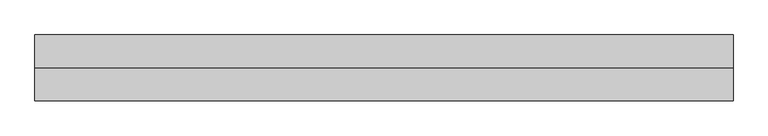
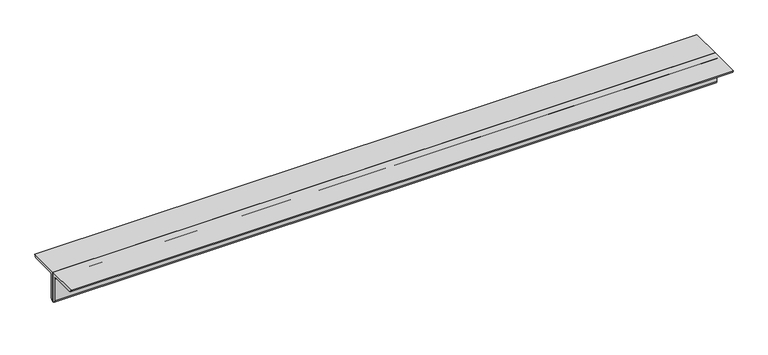
"""IFC4 building model written with IfcOpenShell, lengths in millimetres: beam geometry, 0123_Steel Framing_2Ls-KSD3502 : H_SB_AR_S04_2Ls-130x130x12_VBR1."""

from ifc_helpers import new_model, si_unit, point, frame, frame_2d, origin, place, context, project, spatial, polyline, circle_curve, trimmed, segment, composite_curve, outline, extrude, source, transform, mapped, element, save


def beam_630e65bb(model_context):
    return source(origin(), model_context, "Body", "SweptSolid", [
        extrude(outline(composite_curve([segment(polyline([(0.0, 36.4), (130.0, 36.4)]), True, "CONTINUOUS"), segment(trimmed(circle_curve(frame_2d((118.0, 36.4)), 12.0), [point((130.0, 36.4))], [point((118.0, 24.4))], False, "CARTESIAN"), True, "CONTINUOUS"), segment(polyline([(118.0, 24.4), (24.0, 24.4)]), True, "CONTINUOUS"), segment(trimmed(circle_curve(frame_2d((24.0, 12.4)), 12.0), [point((24.0, 24.4))], [point((12.0, 12.4))], True, "CARTESIAN"), True, "CONTINUOUS"), segment(polyline([(12.0, 12.4), (12.0, -81.6)]), True, "CONTINUOUS"), segment(trimmed(circle_curve(frame_2d((0.0, -81.6)), 12.0), [point((12.0, -81.6))], [point((0.0, -93.6))], False, "CARTESIAN"), True, "CONTINUOUS"), segment(polyline([(0.0, -93.6), (0.0, 36.4)]), True, "CONTINUOUS")], self_intersect=False)), frame((-1375.4177251, 0.0, 0.0), z_axis=(1.0, 0.0, 0.0), x_axis=(0.0, 1.0, 0.0)), (0.0, 0.0, 1.0), 2750.8354501),
        extrude(outline(composite_curve([segment(polyline([(0.0, 36.4), (0.0, -93.6)]), True, "CONTINUOUS"), segment(trimmed(circle_curve(frame_2d((0.0, -81.6)), 12.0), [point((0.0, -93.6))], [point((-12.0, -81.6))], False, "CARTESIAN"), True, "CONTINUOUS"), segment(polyline([(-12.0, -81.6), (-12.0, 12.4)]), True, "CONTINUOUS"), segment(trimmed(circle_curve(frame_2d((-24.0, 12.4)), 12.0), [point((-12.0, 12.4))], [point((-24.0, 24.4))], True, "CARTESIAN"), True, "CONTINUOUS"), segment(polyline([(-24.0, 24.4), (-118.0, 24.4)]), True, "CONTINUOUS"), segment(trimmed(circle_curve(frame_2d((-118.0, 36.4)), 12.0), [point((-118.0, 24.4))], [point((-130.0, 36.4))], False, "CARTESIAN"), True, "CONTINUOUS"), segment(polyline([(-130.0, 36.4), (0.0, 36.4)]), True, "CONTINUOUS")], self_intersect=False)), frame((-1375.4177251, 0.0, 0.0), z_axis=(1.0, 0.0, 0.0), x_axis=(0.0, 1.0, 0.0)), (0.0, 0.0, 1.0), 2750.8354501),
    ])


if __name__ == "__main__":
    model = new_model("IFC4")
    model_context = context("Model", 3, world=origin())
    ifc_project = project(units=[si_unit("LENGTHUNIT", "METRE", prefix="MILLI")], contexts=[model_context])
    site = spatial("IfcSite", under=ifc_project)
    building = spatial("IfcBuilding", under=site)
    placement = place(None, origin())
    beam_shape = beam_630e65bb(model_context)
    element("IfcBeam", 1, ObjectType="0123_Steel Framing_2Ls-KSD3502 : H_SB_AR_S04_2Ls-130x130x12_VBR1", at=placement, inside=building, context=model_context, shape_type="MappedRepresentation", body=[
        mapped(beam_shape, transform((0.0, 0.0, 0.0), x_axis=(1.0, 0.0, 0.0), y_axis=(0.0, 1.0, 0.0), z_axis=(0.0, 0.0, 1.0))),
    ])
    save(model, "model.ifc")

# Revit data of these elements
# Type "0123_Steel Framing_2Ls-KSD3502 : H_SB_AR_S04_2Ls-130x130x12_VBR1"
#   Type Mark = "VBR1"
#   Assembly Code = "B10"
#   Legs = "SLBB"
#   W = 8.97
#   Perimeter = 1.04 m²/m
#   Nominal Weight = 46.80 kgf/m
#   Length [instance default] = 1000 mm
#   Space = 0 mm
#   b = 130 mm
#   d = 130 mm
#   t = 12 mm
#   y = 36.4 mm
#   A = 0.005952 m²
#   Structural Material [instance default] = Steel ASTM A36
# Element 1 (IfcBeam, "0123_Steel Framing_2Ls-KSD3502 : H_SB_AR_S04_2Ls-130x130x12_VBR1")
#   Materials on its faces: "Steel ASTM A36"
# Materials
#   "Steel ASTM A36": class "Metal", colour RGB 199 199 199, transparency 0, Description = "Structural steel, ASTM A36 Grade B, mill finish", Cost = 0
